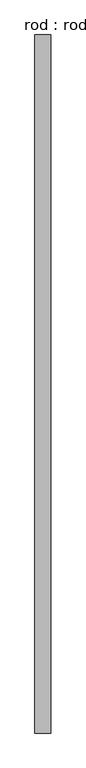
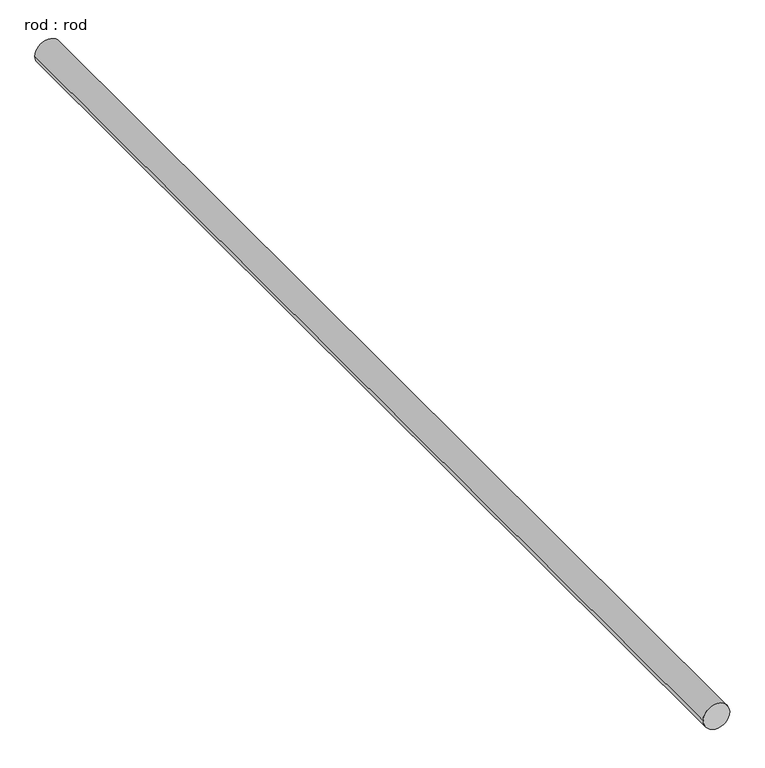
"""IFC4 building model written with IfcOpenShell, lengths in millimetres: proxy geometry, rod : rod."""

from ifc_helpers import new_model, si_unit, point, frame, frame_2d, origin, place, context, project, spatial, circle_curve, trimmed, segment, composite_curve, outline, extrude, source, transform, mapped, element, save


def rod_rod_53a305b0(model_context):
    return source(origin(), model_context, "Body", "SweptSolid", [
        extrude(outline(composite_curve([segment(trimmed(circle_curve(frame_2d((0.0108462, 0.0)), 200.0), [point((0.0108462, 200.0))], [point((0.0108462, -200.0))], False, "CARTESIAN"), True, "CONTINUOUS"), segment(trimmed(circle_curve(frame_2d((0.0108462, 0.0)), 200.0), [point((0.0108462, -200.0))], [point((0.0108462, 200.0))], False, "CARTESIAN"), True, "CONTINUOUS")], self_intersect=False)), frame((0.0, -4657.2713847, 0.0), z_axis=(0.0, 1.0, 0.0), x_axis=(0.0, 0.0, 1.0)), (0.0, 0.0, 1.0), 17500.0),
    ])


if __name__ == "__main__":
    model = new_model("IFC4")
    model_context = context("Model", 3, world=origin())
    ifc_project = project(units=[si_unit("LENGTHUNIT", "METRE", prefix="MILLI")], contexts=[model_context])
    site = spatial("IfcSite", under=ifc_project)
    building = spatial("IfcBuilding", under=site)
    placement = place(None, origin())
    rod_rod_shape = rod_rod_53a305b0(model_context)
    element("IfcBuildingElementProxy", 1, Name="rod : rod", ObjectType="rod : rod", at=placement, inside=building, context=model_context, shape_type="MappedRepresentation", body=[
        mapped(rod_rod_shape, transform((0.0, 0.0, 0.0), x_axis=(1.0, 0.0, 0.0), y_axis=(0.0, 1.0, 0.0), z_axis=(0.0, 0.0, 1.0))),
    ])
    save(model, "model.ifc")

# Revit data of these elements
# Type "rod : rod"
#   Default Elevation = 0
